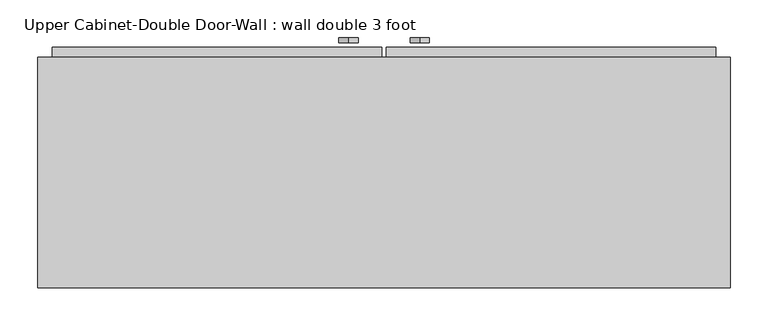
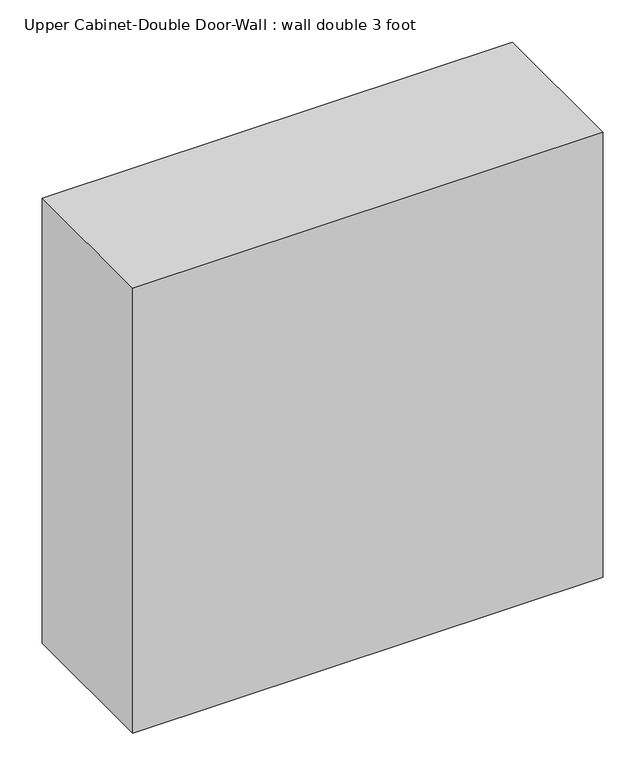
"""IFC4 building model written with IfcOpenShell, lengths in millimetres: furniture geometry, Upper Cabinet-Double Door-Wall : wall double 3 foot."""

from ifc_helpers import new_model, si_unit, point, frame, frame_2d, origin, place, context, project, spatial, polyline, circle_curve, trimmed, segment, composite_curve, outline, extrude, faceted_brep, source, transform, mapped, element, save


def upper_cabinet_double_door_wall_wall_double_3_foot_53664c12(model_context):
    return source(origin(), model_context, "Body", "SolidModel", [
        faceted_brep([(-427.4288372, 56.35625, 2133.6), (-427.4288372, 56.35625, 1219.2), (486.9711628, 56.35625, 1219.2), (486.9711628, 56.35625, 2133.6), (-427.4288372, 361.15625, 2133.6), (486.9711628, 361.15625, 2133.6), (486.9711628, 361.15625, 1219.2), (-427.4288372, 361.15625, 1219.2), (-408.3788372, 361.15625, 2114.55), (-408.3788372, 361.15625, 1238.25), (467.9211628, 361.15625, 1238.25), (467.9211628, 361.15625, 2114.55), (467.9211628, 75.40625, 2114.55), (-408.3788372, 75.40625, 2114.55), (467.9211628, 75.40625, 1238.25), (-408.3788372, 75.40625, 1238.25)], [[[0, 1, 2, 3]], [[4, 5, 6, 7], [8, 9, 10, 11]], [[1, 0, 4, 7]], [[2, 1, 7, 6]], [[3, 2, 6, 5]], [[0, 3, 5, 4]], [[8, 11, 12, 13]], [[11, 10, 14, 12]], [[10, 9, 15, 14]], [[9, 8, 13, 15]], [[13, 12, 14, 15]]]),
        extrude(outline(polyline([(32.9461628, 373.85625), (467.9211628, 373.85625), (467.9211628, 342.10625), (32.9461628, 342.10625), (32.9461628, 373.85625)])), frame((0.0, 0.0, 1238.25), z_axis=(0.0, 0.0, 1.0), x_axis=(1.0, 0.0, 0.0)), (0.0, 0.0, 1.0), 876.3),
        extrude(outline(polyline([(-408.3788372, 373.85625), (26.5961628, 373.85625), (26.5961628, 342.10625), (-408.3788372, 342.10625), (-408.3788372, 373.85625)])), frame((0.0, 0.0, 1238.25), z_axis=(0.0, 0.0, 1.0), x_axis=(1.0, 0.0, 0.0)), (0.0, 0.0, 1.0), 876.3),
        extrude(outline(composite_curve([segment(trimmed(circle_curve(frame_2d((1381.4214732, 76.8007051)), 12.7), [point((1368.7214732, 76.8007051))], [point((1394.1214732, 76.8007051))], False, "CARTESIAN"), True, "CONTINUOUS"), segment(trimmed(circle_curve(frame_2d((1381.4214732, 76.8007051)), 12.7), [point((1394.1214732, 76.8007051))], [point((1368.7214732, 76.8007051))], False, "CARTESIAN"), True, "CONTINUOUS")], self_intersect=False)), frame((0.0, 380.20625, 0.0), z_axis=(0.0, 1.0, 0.0), x_axis=(0.0, 0.0, 1.0)), (0.0, 0.0, 1.0), 6.35),
        extrude(outline(composite_curve([segment(trimmed(circle_curve(frame_2d((1381.4214732, -17.2583796)), 12.7), [point((1368.7214732, -17.2583796))], [point((1394.1214732, -17.2583796))], False, "CARTESIAN"), True, "CONTINUOUS"), segment(trimmed(circle_curve(frame_2d((1381.4214732, -17.2583796)), 12.7), [point((1394.1214732, -17.2583796))], [point((1368.7214732, -17.2583796))], False, "CARTESIAN"), True, "CONTINUOUS")], self_intersect=False)), frame((0.0, 380.20625, 0.0), z_axis=(0.0, 1.0, 0.0), x_axis=(0.0, 0.0, 1.0)), (0.0, 0.0, 1.0), 6.35),
    ])


if __name__ == "__main__":
    model = new_model("IFC4")
    model_context = context("Model", 3, world=origin())
    ifc_project = project(units=[si_unit("LENGTHUNIT", "METRE", prefix="MILLI")], contexts=[model_context])
    site = spatial("IfcSite", under=ifc_project)
    building = spatial("IfcBuilding", under=site)
    placement = place(None, origin())
    upper_cabinet_double_door_wall_wall_double_3_foot_shape = upper_cabinet_double_door_wall_wall_double_3_foot_53664c12(model_context)
    element("IfcFurniture", 1, ObjectType="Upper Cabinet-Double Door-Wall : wall double 3 foot", at=placement, inside=building, context=model_context, shape_type="MappedRepresentation", body=[
        mapped(upper_cabinet_double_door_wall_wall_double_3_foot_shape, transform((0.0, 0.0, 0.0), x_axis=(1.0, 0.0, 0.0), y_axis=(0.0, 1.0, 0.0), z_axis=(0.0, 0.0, 1.0))),
    ])
    save(model, "model.ifc")

# Revit data of these elements
# Type "Upper Cabinet-Double Door-Wall : wall double 3 foot"
#   Assembly Code = "C1030410"
#   Depth = 1' - 0"
#   Height = 3' - 0"
#   Top Of Cabinet = 7' - 0"
#   Width = 3' - 0"
#   Cabinet Material = Base cabinet 2120100 Aspekt - 83012120100 - White
#   Door/Drawer Material = Base cabinet 2120100 Aspekt - 83012120100 - White
#   Handle Material = Cabinets - Handles
#   Default Elevation = 0
# Element 1 (IfcFurniture, "Upper Cabinet-Double Door-Wall : wall double 3 foot")
#   Materials on its faces: "Base cabinet 2120100 Aspekt - 83012120100 - White"
# Materials
#   "Base cabinet 2120100 Aspekt - 83012120100 - White": class "Miscellaneous", colour RGB 255 255 255, transparency 0, Manufacturer = "Marbodal", URL = "http://www.marbodal.se", Cost = 0
#   "Cabinets - Handles": class "Metal", colour RGB 57 57 57, transparency 0
